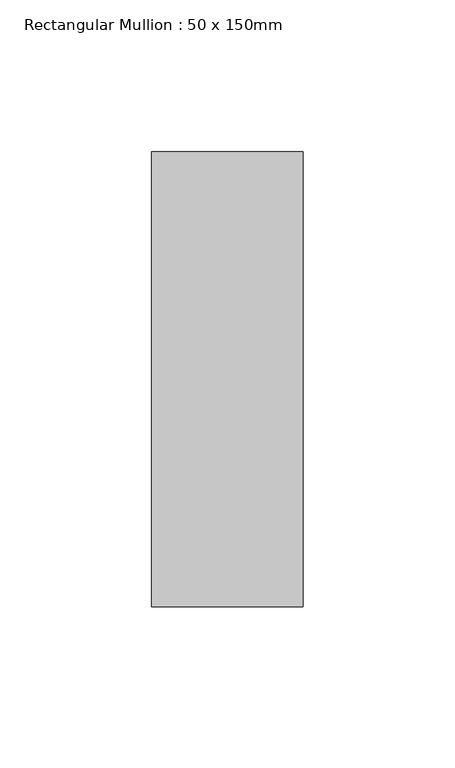
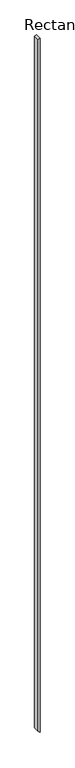
"""IFC4 building model written with IfcOpenShell, lengths in millimetres: member geometry, Rectangular Mullion : 50 x 150mm."""

from ifc_helpers import new_model, si_unit, frame, origin, place, context, project, spatial, polyline, outline, extrude, source, transform, mapped, element, save


def rectangular_mullion_50_x_150mm_3d894c4c(model_context):
    return source(origin(), model_context, "Body", "SweptSolid", [
        extrude(outline(polyline([(0.0, 0.0), (-16.6341861, -50.0), (-17948.6640858, -50.0), (-17995.7375779, 0.0), (0.0, 0.0)])), frame((0.0, -75.0, 0.0), z_axis=(0.0, 1.0, 0.0), x_axis=(0.0, 0.0, 1.0)), (0.0, 0.0, 1.0), 150.0),
    ])


if __name__ == "__main__":
    model = new_model("IFC4")
    model_context = context("Model", 3, world=origin())
    ifc_project = project(units=[si_unit("LENGTHUNIT", "METRE", prefix="MILLI")], contexts=[model_context])
    site = spatial("IfcSite", under=ifc_project)
    building = spatial("IfcBuilding", under=site)
    placement = place(None, origin())
    rectangular_mullion_50_x_150mm_shape = rectangular_mullion_50_x_150mm_3d894c4c(model_context)
    element("IfcMember", 1, ObjectType="Rectangular Mullion : 50 x 150mm", at=placement, inside=building, context=model_context, shape_type="MappedRepresentation", body=[
        mapped(rectangular_mullion_50_x_150mm_shape, transform((0.0, 0.0, 0.0), x_axis=(1.0, 0.0, 0.0), y_axis=(0.0, 1.0, 0.0), z_axis=(0.0, 0.0, 1.0))),
    ])
    save(model, "model.ifc")

# Revit data of these elements
# Type "Rectangular Mullion : 50 x 150mm"
#   built-in parameter 1007304 = 0.492126 (stored number, unit not read)
#   built-in parameter 1007301 = 0.082021 (stored number, unit not read)
#   built-in parameter 1007300 = 0.082021 (stored number, unit not read)
# Element 1 (IfcMember, "Rectangular Mullion : 50 x 150mm")
#   Materials on its faces: "Metal - Aluminium"
# Materials
#   "Metal - Aluminium": class "Metal", colour RGB 247 247 247, transparency 0
